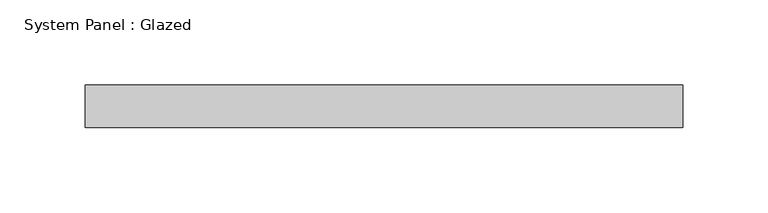
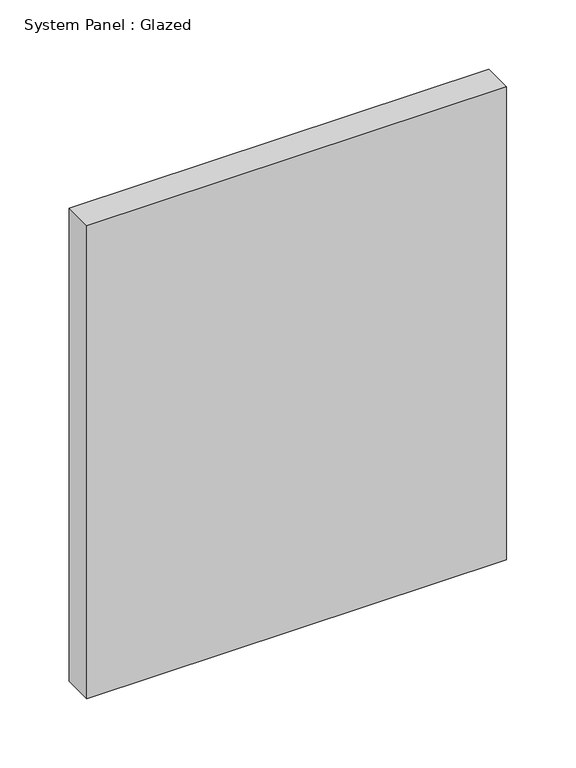
"""IFC4 building model written with IfcOpenShell, lengths in millimetres: plate geometry, System Panel : Glazed."""

import ifcopenshell
import ifcopenshell.guid

model = None  # the IFC model being written
_history = None  # IfcOwnerHistory: only IFC2X3 demands one
_inside = {}  # id of a spatial element -> (the spatial element, [elements in it])
_under = {}  # id of a project, library or spatial element -> (it, [spatial elements below it])
_declared = {}  # id of a project -> (the project, [libraries it declares])
_typed = {}  # id of a type object -> (the type object, [elements of that type])
_made_of = {}  # id of a material, layer set ... -> (it, [elements and type objects made of it])


def new_model(schema):
    """Start an empty IFC model of exactly this schema.

    Asked for "IFC4X3", IfcOpenShell would pick the latest addendum, in which some entities
    have other attributes; the version numbers below select the first issue.
    IFC2X3 requires an IfcOwnerHistory on every rooted entity: one is made here for all.
    """
    global model, _history
    if schema == "IFC4X3":
        model = ifcopenshell.file(schema_version=(4, 3, 0, 0))
    else:
        model = ifcopenshell.file(schema=schema)
    _inside.clear()
    _under.clear()
    _declared.clear()
    _typed.clear()
    _made_of.clear()
    _history = None
    if model.schema == "IFC2X3":
        org = make("IfcOrganization", Name="unknown")
        user = make(
            "IfcPersonAndOrganization",
            ThePerson=make("IfcPerson", FamilyName="unknown"),
            TheOrganization=org,
        )
        app = make(
            "IfcApplication",
            ApplicationDeveloper=org,
            Version="unknown",
            ApplicationFullName="unknown",
            ApplicationIdentifier="unknown",
        )
        _history = make(
            "IfcOwnerHistory",
            OwningUser=user,
            OwningApplication=app,
            ChangeAction="ADDED",
            CreationDate=0,
        )
    return model


def make(cls, **values):
    """One entity of the class cls with the attributes given. An attribute that is None is left unset."""
    return model.create_entity(
        cls, **{name: value for name, value in values.items() if value is not None}
    )


def rooted(cls, **values):
    """An entity with a GlobalId (a new one), such as an element, a storey or a relation."""
    return make(cls, GlobalId=ifcopenshell.guid.new(), OwnerHistory=_history, **values)


def si_unit(unit_type, name, prefix=None):
    """IfcSIUnit, for example si_unit("LENGTHUNIT", "METRE", prefix="MILLI")."""
    return make("IfcSIUnit", UnitType=unit_type, Prefix=prefix, Name=name)


def assignment(units):
    """IfcUnitAssignment: the units of a project."""
    return None if units is None else make("IfcUnitAssignment", Units=units)


def point(xyz):
    """IfcCartesianPoint."""
    return None if xyz is None else make("IfcCartesianPoint", Coordinates=xyz)


def direction(xyz):
    """IfcDirection."""
    return None if xyz is None else make("IfcDirection", DirectionRatios=xyz)


def frame(location, z_axis=None, x_axis=None):
    """IfcAxis2Placement3D, a coordinate frame: its origin and axes. An axis left out is left unset."""
    return make(
        "IfcAxis2Placement3D",
        Location=point(location),
        Axis=direction(z_axis),
        RefDirection=direction(x_axis),
    )


def origin():
    """The frame at (0, 0, 0) with its axes left unset."""
    return frame((0.0, 0.0, 0.0))


def origin_with_axes():
    """The frame at (0, 0, 0) with the z axis (0, 0, 1) and the x axis (1, 0, 0) written out."""
    return frame((0.0, 0.0, 0.0), z_axis=(0.0, 0.0, 1.0), x_axis=(1.0, 0.0, 0.0))


def place(relative_to, where):
    """IfcLocalPlacement: puts the frame where relative to a parent placement (None: the world)."""
    return make(
        "IfcLocalPlacement", PlacementRelTo=relative_to, RelativePlacement=where
    )


def context(
    kind, dimensions, precision=None, world=None, true_north=None, identifier=None
):
    """IfcGeometricRepresentationContext, for example the 3D "Model" context."""
    return make(
        "IfcGeometricRepresentationContext",
        ContextIdentifier=identifier,
        ContextType=kind,
        CoordinateSpaceDimension=dimensions,
        Precision=precision,
        WorldCoordinateSystem=world,
        TrueNorth=true_north,
    )


def project(units=None, contexts=None):
    """IfcProject with its units and contexts."""
    return rooted(
        "IfcProject",
        Name="project",
        RepresentationContexts=contexts,
        UnitsInContext=assignment(units),
    )


def spatial(cls, under=None, at=None, **own):
    """A site, building, storey or space (cls), placed at a placement, below another one or the project."""
    s = rooted(cls, ObjectPlacement=at, **own)
    if under is not None:
        _under.setdefault(under.id(), (under, []))[1].append(s)
    return s


def polyline(points):
    """IfcPolyline through the points."""
    return make("IfcPolyline", Points=[point(p) for p in points])


def outline(outer, holes=None, kind="AREA"):
    """IfcArbitraryClosedProfileDef: a profile drawn as a closed curve; with holes, ...WithVoids."""
    if holes is None:
        return make("IfcArbitraryClosedProfileDef", ProfileType=kind, OuterCurve=outer)
    return make(
        "IfcArbitraryProfileDefWithVoids",
        ProfileType=kind,
        OuterCurve=outer,
        InnerCurves=holes,
    )


def extrude(swept, where, along, depth):
    """IfcExtrudedAreaSolid: the profile swept, set in the frame where, extruded along a direction by depth."""
    return make(
        "IfcExtrudedAreaSolid",
        SweptArea=swept,
        Position=where,
        ExtrudedDirection=direction(along),
        Depth=depth,
    )


def shape(context_of_items, identifier, shape_type, items):
    """IfcShapeRepresentation: the items that make up one representation, for example the "Body"."""
    return make(
        "IfcShapeRepresentation",
        ContextOfItems=context_of_items,
        RepresentationIdentifier=identifier,
        RepresentationType=shape_type,
        Items=items,
    )


def source(mapping_origin, context_of_items, identifier, shape_type, items):
    """IfcRepresentationMap: a shape defined once, which mapped items show again and again."""
    return make(
        "IfcRepresentationMap",
        MappingOrigin=mapping_origin,
        MappedRepresentation=shape(context_of_items, identifier, shape_type, items),
    )


def transform(
    local_origin,
    x_axis=None,
    y_axis=None,
    z_axis=None,
    scale=None,
    scale2=None,
    scale3=None,
    uniform=True,
):
    """IfcCartesianTransformationOperator3D, or its non-uniform kind. x_axis, y_axis, z_axis: its Axis1, 2, 3."""
    if uniform:
        return make(
            "IfcCartesianTransformationOperator3D",
            Axis1=direction(x_axis),
            Axis2=direction(y_axis),
            LocalOrigin=point(local_origin),
            Scale=scale,
            Axis3=direction(z_axis),
        )
    return make(
        "IfcCartesianTransformationOperator3DnonUniform",
        Axis1=direction(x_axis),
        Axis2=direction(y_axis),
        LocalOrigin=point(local_origin),
        Scale=scale,
        Axis3=direction(z_axis),
        Scale2=scale2,
        Scale3=scale3,
    )


def mapped(mapping_source, mapping_target):
    """IfcMappedItem: shows the shape of a source again, moved by a transform."""
    return make(
        "IfcMappedItem", MappingSource=mapping_source, MappingTarget=mapping_target
    )


def made_of(thing, what):
    """Note that an element or type object is made of a material, layer set ...; save() writes the relation."""
    if what is not None:
        _made_of.setdefault(what.id(), (what, []))[1].append(thing)
    return thing


def element(
    cls,
    number,
    at=None,
    inside=None,
    cuts=None,
    type_object=None,
    material=None,
    context=None,
    identifier="Body",
    shape_type=None,
    held_by="IfcProductDefinitionShape",
    body=None,
    shapes=None,
    **own,
):
    """One element of the class cls, such as IfcWall. Its Tag is "e" and its number.

    at: its placement. inside: the storey or other place that contains it. cuts: it is an
    opening in that element (IfcRelVoidsElement). A single representation is given by context,
    identifier, shape_type and body (its items); several are given by shapes. held_by: the class
    of the entity that holds the representations. save() writes the other relations.
    """
    e = rooted(cls, Tag="e%d" % number, ObjectPlacement=at, **own)
    if body is not None:
        shapes = [shape(context, identifier, shape_type, body)]
    if shapes is not None:
        e.Representation = make(held_by, Representations=shapes)
    if inside is not None:
        _inside.setdefault(inside.id(), (inside, []))[1].append(e)
    if cuts is not None:
        rooted(
            "IfcRelVoidsElement", RelatingBuildingElement=cuts, RelatedOpeningElement=e
        )
    if type_object is not None:
        _typed.setdefault(type_object.id(), (type_object, []))[1].append(e)
    return made_of(e, material)


def aggregate(whole, parts):
    """IfcRelAggregates: a whole, such as a stair, and the parts it consists of."""
    return rooted("IfcRelAggregates", RelatingObject=whole, RelatedObjects=parts)


def save(model, path):
    """Write the relations noted so far, then the file.

    IfcRelAggregates (storeys below a building ...), IfcRelContainedInSpatialStructure (elements
    in a storey), IfcRelDefinesByType, IfcRelAssociatesMaterial and IfcRelDeclares: one each for
    every whole, place, type object, material and project.
    """
    for whole, parts in _under.values():
        aggregate(whole, parts)
    for where, things in _inside.values():
        rooted(
            "IfcRelContainedInSpatialStructure",
            RelatedElements=things,
            RelatingStructure=where,
        )
    for kind, things in _typed.values():
        rooted("IfcRelDefinesByType", RelatedObjects=things, RelatingType=kind)
    for what, things in _made_of.values():
        rooted("IfcRelAssociatesMaterial", RelatedObjects=things, RelatingMaterial=what)
    for by, libraries in _declared.values():
        rooted("IfcRelDeclares", RelatingContext=by, RelatedDefinitions=libraries)
    model.write(path)


def system_panel_glazed_12acb79b(model_context):
    return source(origin(), model_context, "Body", "SweptSolid", [
        extrude(outline(polyline([(175.0, 24.5), (-175.0, 24.5), (-175.0, 49.5), (175.0, 49.5), (175.0, 24.5)])), origin_with_axes(), (0.0, 0.0, 1.0), 416.6666667),
    ])


if __name__ == "__main__":
    model = new_model("IFC4")
    model_context = context("Model", 3, world=origin())
    ifc_project = project(units=[si_unit("LENGTHUNIT", "METRE", prefix="MILLI")], contexts=[model_context])
    site = spatial("IfcSite", under=ifc_project)
    building = spatial("IfcBuilding", under=site)
    placement = place(None, origin())
    system_panel_glazed_shape = system_panel_glazed_12acb79b(model_context)
    element("IfcPlate", 1, ObjectType="System Panel : Glazed", at=placement, inside=building, context=model_context, shape_type="MappedRepresentation", body=[
        mapped(system_panel_glazed_shape, transform((0.0, 0.0, 0.0), x_axis=(1.0, 0.0, 0.0), y_axis=(0.0, 1.0, 0.0), z_axis=(0.0, 0.0, 1.0))),
    ])
    save(model, "model.ifc")

# Revit data of these elements
# Element 1 (IfcPlate, "System Panel : Glazed")
#   Materials on its faces: "Glass"
# Materials
#   "Glass": class "Glass", colour RGB 218 227 224, transparency 0.85, Description = "Soda Lime Glass", Cost = 0
